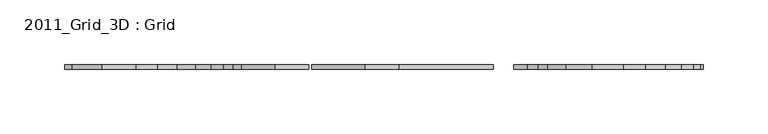
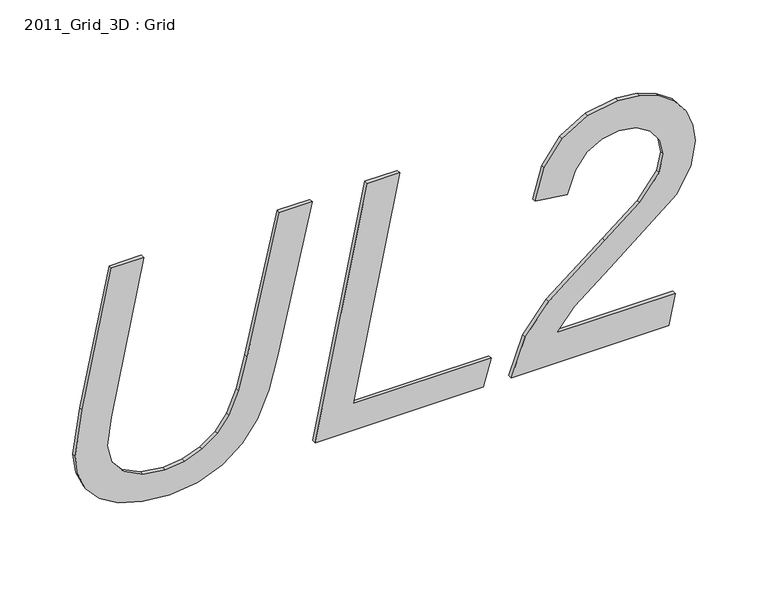
"""IFC4 building model written with IfcOpenShell, lengths in millimetres: proxy geometry, 2011_Grid_3D : Grid."""

from ifc_helpers import new_model, si_unit, frame, origin, place, context, project, spatial, polyline, outline, extrude, source, transform, mapped, element, save


def proxy_2011_grid_3d_grid_3a42ab4e(model_context):
    return source(origin(), model_context, "Body", "SweptSolid", [
        extrude(outline(polyline([(101.4447294, 32343.9093434), (-9.5457855, 32320.8090397), (-46.3278141, 32315.1578924), (-62.2836301, 32317.3018584), (-76.4424804, 32323.7337562), (-88.2714718, 32334.4659789), (-97.2377109, 32349.5109192), (-102.8888581, 32368.2985052), (-104.7725739, 32390.2586651), (-102.1081075, 32412.4542896), (-94.1147085, 32431.7499831), (-81.7032524, 32447.6500312), (-65.784615, 32459.6587191), (-44.9584024, 32468.7550833), (-17.8242205, 32475.9181603), (101.4447294, 32503.0833243), (101.4447294, 32477.157447), (-10.7355007, 32451.57857), (-36.7791103, 32444.8864219), (-54.6310349, 32437.4011304), (-66.7202764, 32428.1064803), (-75.4758368, 32415.9862566), (-80.7923767, 32401.9079599), (-82.5645566, 32386.739091), (-80.0983761, 32368.639309), (-72.6998347, 32353.897994), (-61.2488258, 32344.1014328), (-46.6252429, 32340.8359124), (-23.5745107, 32343.9589148), (101.4447294, 32369.6369348), (101.4447294, 32343.9093434)])), frame((0.0, -3.175, 0.0), z_axis=(0.0, 1.0, 0.0), x_axis=(0.0, 0.0, 1.0)), (0.0, 0.0, 1.0), 3.175),
        extrude(outline(polyline([(-101.6, 32505.5123262), (-101.6, 32638.7604299), (-79.3919827, 32645.1055777), (-79.3919827, 32535.8004926), (101.4447294, 32572.5329498), (101.4447294, 32546.7557869), (-101.6, 32505.5123262)])), frame((0.0, -3.175, 0.0), z_axis=(0.0, 1.0, 0.0), x_axis=(0.0, 0.0, 1.0)), (0.0, 0.0, 1.0), 3.175),
        extrude(outline(polyline([(-101.6, 32660.9684472), (-101.6, 32786.0372587), (-76.2194088, 32791.0439769), (-76.2194088, 32697.1556182), (-59.4146815, 32711.0604147), (-36.6118066, 32739.1922223), (6.8127986, 32792.2336921), (26.1828494, 32803.2385578), (46.3212579, 32806.9068464), (60.1826794, 32805.0974878), (73.6103506, 32799.6694122), (85.3463954, 32790.6412087), (94.132938, 32778.0314668), (99.6167815, 32762.7944371), (101.4447294, 32745.8843704), (97.3302976, 32721.501405), (84.9870023, 32701.4931215), (65.5054157, 32687.2103426), (39.9761101, 32680.0038905), (36.6052504, 32705.3844817), (54.4881571, 32711.6118973), (66.6951309, 32720.9747081), (73.7218864, 32732.8160923), (76.0641382, 32746.479228), (73.7528686, 32760.0927921), (66.8190596, 32771.3888902), (56.5763552, 32778.991914), (44.3383992, 32781.5262552), (29.7643879, 32778.2545384), (9.6879437, 32762.8378121), (-12.2226448, 32735.3256479), (-47.7901724, 32690.5873988), (-71.1135477, 32671.9485271), (-101.6, 32660.9684472)])), frame((0.0, -3.175, 0.0), z_axis=(0.0, 1.0, 0.0), x_axis=(0.0, 0.0, 1.0)), (0.0, 0.0, 1.0), 3.175),
    ])


if __name__ == "__main__":
    model = new_model("IFC4")
    model_context = context("Model", 3, world=origin())
    ifc_project = project(units=[si_unit("LENGTHUNIT", "METRE", prefix="MILLI")], contexts=[model_context])
    site = spatial("IfcSite", under=ifc_project)
    building = spatial("IfcBuilding", under=site)
    placement = place(None, origin())
    proxy_2011_grid_3d_grid_shape = proxy_2011_grid_3d_grid_3a42ab4e(model_context)
    element("IfcBuildingElementProxy", 1, Name="2011_Grid_3D : Grid", ObjectType="2011_Grid_3D : Grid", at=placement, inside=building, context=model_context, shape_type="MappedRepresentation", body=[
        mapped(proxy_2011_grid_3d_grid_shape, transform((0.0, 0.0, 0.0), x_axis=(1.0, 0.0, 0.0), y_axis=(0.0, 1.0, 0.0), z_axis=(0.0, 0.0, 1.0))),
    ])
    save(model, "model.ifc")

# Revit data of these elements
# Type "2011_Grid_3D : Grid"
#   Workplane [instance default] = "LEVEL"
#   Grid [instance default] = "S"
#   t [instance default] = 12' - 6"
#   built-in parameter 1001306 [instance default] = 50 (stored number, unit not read)
#   d [instance default] = 2
#   Symbol At End 2 [instance default] = yes
#   Symbol At End 1 [instance default] = yes
#   Robust [instance default] = yes
#   No of grid markers [instance default] = 3
#   Grid Height Visible = yes
#   Height = 0
#   Assembly Code = ""
# Element 1 (IfcBuildingElementProxy, "2011_Grid_3D : Grid")
#   Workplane = "UL2"
#   Grid = "1"
#   t = 13' - 2.15638"
#   built-in parameter 1001306 = 105.438 (stored number, unit not read)
#   d = 4
#   Robust = no
#   No of grid markers = 5
#   Materials on its faces: "Letter"
# Materials
#   "Letter": class "Unassigned", colour RGB 178 187 30, transparency 0, Comments = "Rendering appearance not upgraded "
